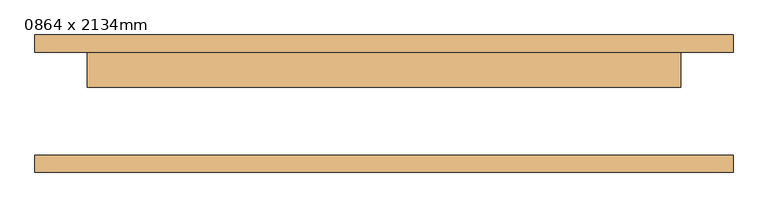
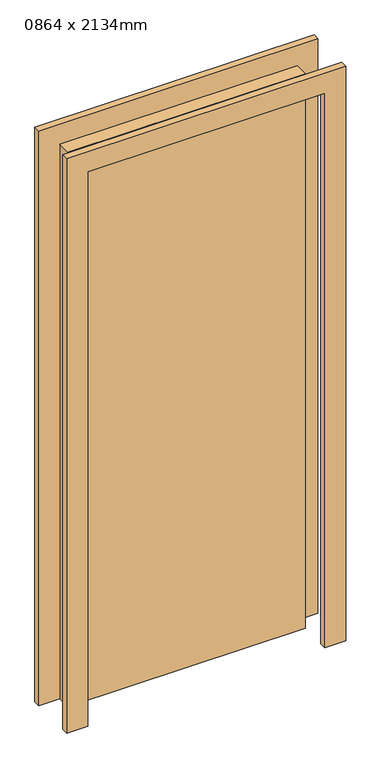
"""IFC4 building model written with IfcOpenShell, lengths in millimetres: door geometry, M_Folha única : 0864 x 2134mm."""

from ifc_helpers import new_model, si_unit, frame, origin, origin_with_axes, place, context, project, spatial, polyline, outline, extrude, source, transform, mapped, element, save


def door_0864_x_2134mm_191ab4f9(model_context):
    return source(origin(), model_context, "Body", "SweptSolid", [
        extrude(outline(polyline([(2210.0, -508.0), (0.0, -508.0), (0.0, -432.0), (2134.0, -432.0), (2134.0, 432.0), (0.0, 432.0), (0.0, 508.0), (2210.0, 508.0), (2210.0, -508.0)])), frame((0.0, 75.0, 0.0), z_axis=(0.0, 1.0, 0.0), x_axis=(0.0, 0.0, 1.0)), (0.0, 0.0, 1.0), 25.0),
        extrude(outline(polyline([(2210.0, 508.0), (2210.0, -508.0), (0.0, -508.0), (0.0, -432.0), (2134.0, -432.0), (2134.0, 432.0), (0.0, 432.0), (0.0, 508.0), (2210.0, 508.0)])), frame((0.0, -100.0, 0.0), z_axis=(0.0, 1.0, 0.0), x_axis=(0.0, 0.0, 1.0)), (0.0, 0.0, 1.0), 25.0),
        extrude(outline(polyline([(432.0, 24.0), (-432.0, 24.0), (-432.0, 75.0), (432.0, 75.0), (432.0, 24.0)])), origin_with_axes(), (0.0, 0.0, 1.0), 2134.0),
    ])


if __name__ == "__main__":
    model = new_model("IFC4")
    model_context = context("Model", 3, world=origin())
    ifc_project = project(units=[si_unit("LENGTHUNIT", "METRE", prefix="MILLI")], contexts=[model_context])
    site = spatial("IfcSite", under=ifc_project)
    building = spatial("IfcBuilding", under=site)
    placement = place(None, origin())
    door_0864_x_2134mm_shape = door_0864_x_2134mm_191ab4f9(model_context)
    element("IfcDoor", 1, ObjectType="M_Folha única : 0864 x 2134mm", at=placement, inside=building, context=model_context, shape_type="MappedRepresentation", body=[
        mapped(door_0864_x_2134mm_shape, transform((0.0, 0.0, 0.0), x_axis=(1.0, 0.0, 0.0), y_axis=(0.0, 1.0, 0.0), z_axis=(0.0, 0.0, 1.0))),
    ])
    save(model, "model.ifc")

# Revit data of these elements
# Type "M_Folha única : 0864 x 2134mm"
#   Type Mark = "22"
#   Construction Type Id = "MDOOR"
#   Analytic Construction = "Metal"
#   Thickness = 0.051 m
#   Thermal Resistance (R) = 0.270117 (m²·K)/W
#   Heat Transfer Coefficient (U) = 3.7021 W/(m²·K)
#   Height = 2.134 m
#   Projeção da apara externa = 0.025 m
#   Projeção da apara interna = 0.025 m
#   Largura da apara = 0.076 m
#   Width = 0.864 m
#   Define Thermal Properties by = 1
#   Material da porta = Porta - Painel
#   Material da moldura = Porta - Batente
#   Visual Light Transmittance = 0
#   Solar Heat Gain Coefficient = 0
#   Function = (empty or 0)
#   Wall Closure = (empty or 0)
# Element 1 (IfcDoor, "M_Folha única : 0864 x 2134mm")
#   Materials on its faces: "Porta - Batente", "Porta - Painel"
# Materials
#   "Porta - Painel": class "Madeira", colour RGB 210 159 95, transparency 0, Cost = 0
#   "Porta - Batente": class "Diversos", colour RGB 118 70 51, transparency 0, Cost = 0
